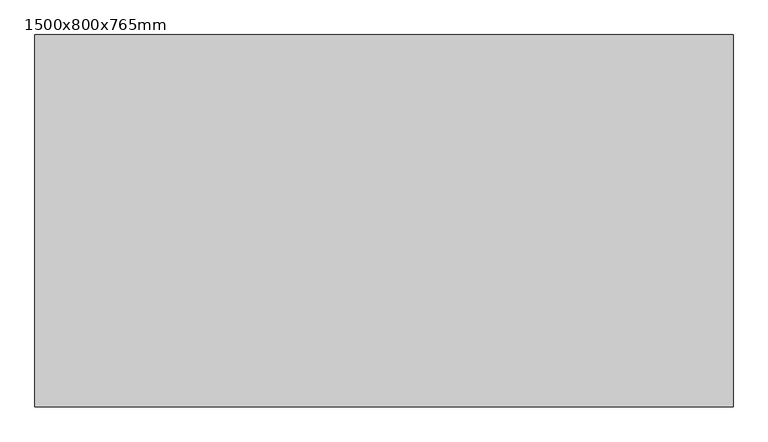
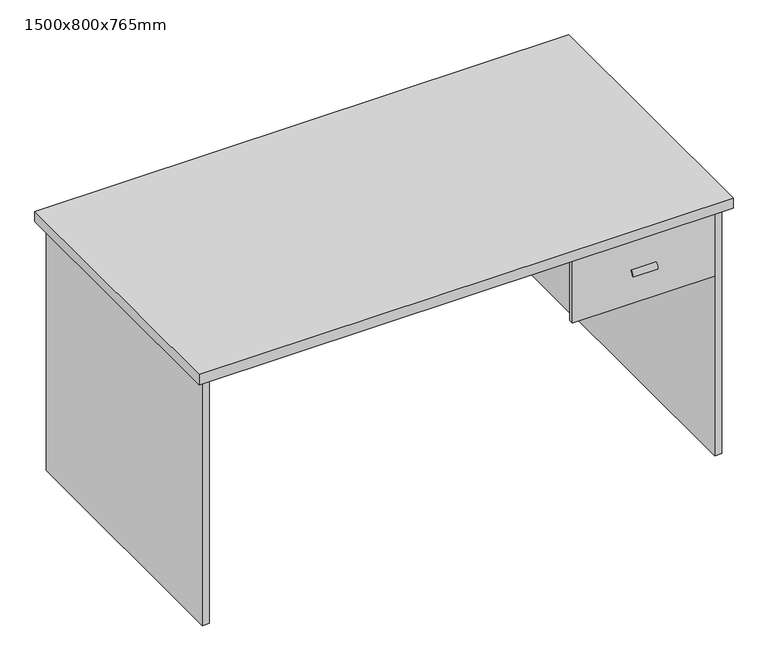
"""IFC4 building model written with IfcOpenShell, lengths in millimetres: furniture geometry, NBS_OffcDsks_OfficeDeskWithDrawer : 1500x800x765mm."""

from ifc_helpers import new_model, si_unit, point, frame, frame_2d, origin, origin_with_axes, place, context, project, spatial, polyline, circle_curve, trimmed, segment, composite_curve, outline, extrude, source, transform, mapped, element, save


def furniture_1500x800x765mm_9c7e9ddd(model_context):
    return source(origin(), model_context, "Body", "SweptSolid", [
        extrude(outline(polyline([(710.0, -380.0), (310.0, -380.0), (310.0, -368.0), (710.0, -368.0), (710.0, -380.0)])), frame((0.0, 0.0, 535.0), z_axis=(0.0, 0.0, 1.0), x_axis=(1.0, 0.0, 0.0)), (0.0, 0.0, 1.0), 200.0),
        extrude(outline(polyline([(698.0, 60.0), (698.0, -368.0), (321.9992987, -368.0), (321.9992987, 60.0), (698.0, 60.0)])), frame((0.0, 0.0, 540.7416159), z_axis=(0.0, 0.0, 1.0), x_axis=(1.0, 0.0, 0.0)), (0.0, 0.0, 1.0), 194.2583841),
        extrude(outline(polyline([(710.0, 380.0), (710.0, 360.0), (-710.0, 360.0), (-710.0, 380.0), (710.0, 380.0)])), frame((0.0, 0.0, 185.0), z_axis=(0.0, 0.0, 1.0), x_axis=(1.0, 0.0, 0.0)), (0.0, 0.0, 1.0), 550.0),
        extrude(outline(polyline([(-710.0, 380.0), (-710.0, -380.0), (-730.0, -380.0), (-730.0, 380.0), (-710.0, 380.0)])), origin_with_axes(), (0.0, 0.0, 1.0), 735.0),
        extrude(outline(polyline([(730.0, 380.0), (730.0, -380.0), (710.0, -380.0), (710.0, 380.0), (730.0, 380.0)])), origin_with_axes(), (0.0, 0.0, 1.0), 735.0),
        extrude(outline(polyline([(750.0, 400.0), (750.0, -400.0), (-750.0, -400.0), (-750.0, 400.0), (750.0, 400.0)])), frame((0.0, 0.0, 735.0), z_axis=(0.0, 0.0, 1.0), x_axis=(1.0, 0.0, 0.0)), (0.0, 0.0, 1.0), 30.0),
        extrude(outline(composite_curve([segment(trimmed(circle_curve(frame_2d((-369.1756558, 618.6602663)), 20.2222385), [point((-389.3776536, 619.5648197))], [point((-380.0, 635.7416159))], False, "CARTESIAN"), True, "CONTINUOUS"), segment(polyline([(-380.0, 635.7416159), (-380.0, 631.5709177)]), True, "CONTINUOUS"), segment(trimmed(circle_curve(frame_2d((-367.0301873, 617.1513707)), 19.394313), [point((-380.0, 631.5709177))], [point((-384.452251, 625.6725838))], True, "CARTESIAN"), True, "CONTINUOUS"), segment(trimmed(circle_curve(frame_2d((-393.0621605, 627.5759127)), 8.8177776), [point((-384.452251, 625.6725838))], [point((-389.3776536, 619.5648197))], False, "CARTESIAN"), True, "CONTINUOUS")], self_intersect=False)), frame((475.0, 0.0, 0.0), z_axis=(1.0, 0.0, 0.0), x_axis=(0.0, 1.0, 0.0)), (0.0, 0.0, 1.0), 70.0),
    ])


if __name__ == "__main__":
    model = new_model("IFC4")
    model_context = context("Model", 3, world=origin())
    ifc_project = project(units=[si_unit("LENGTHUNIT", "METRE", prefix="MILLI")], contexts=[model_context])
    site = spatial("IfcSite", under=ifc_project)
    building = spatial("IfcBuilding", under=site)
    placement = place(None, origin())
    furniture_1500x800x765mm_shape = furniture_1500x800x765mm_9c7e9ddd(model_context)
    element("IfcFurniture", 1, ObjectType="NBS_OffcDsks_OfficeDeskWithDrawer : 1500x800x765mm", at=placement, inside=building, context=model_context, shape_type="MappedRepresentation", body=[
        mapped(furniture_1500x800x765mm_shape, transform((0.0, 0.0, 0.0), x_axis=(1.0, 0.0, 0.0), y_axis=(0.0, 1.0, 0.0), z_axis=(0.0, 0.0, 1.0))),
    ])
    save(model, "model.ifc")

# Revit data of these elements
# Type "NBS_OffcDsks_OfficeDeskWithDrawer : 1500x800x765mm"
#   Type IfcGUID = "2u0XNFrAPALBFZCv81fq27"
#   WarrantyStartDate [instance default] = "1900-12-31T23:59:59"
#   WarrantyGuarantorParts = "n/a"
#   WarrantyGuarantorLabor = "n/a"
#   WarrantyDurationUnit = "year"
#   WarrantyDurationParts = "n/a"
#   WarrantyDurationLabor = "n/a"
#   WarrantyDescription = "n/a"
#   Version = "2"
#   Uniclass2015Version = "Products v1.9"
#   Uniclass2015Title = "Office desks"
#   Uniclass2015Code = "Pr_40_50_21_59"
#   URL = "www.nationalbimlibrary.com"
#   TagNumber [instance default] = "n/a"
#   SustainabilityPerformance = "n/a"
#   Style = "n/a"
#   Size = "1500 x 800 x 765 mm"
#   Shape = "n/a"
#   SerialNumber [instance default] = "n/a"
#   Revision = "n/a"
#   ReplacementCost = "n/a"
#   ProductInformation = "www.nationalbimlibrary.com"
#   OmniClassVersion = "Table 22 2012-05-16"
#   OmniClassTitle = "Office Tables"
#   OmniClassCode = "22-12 51 23"
#   Name = "OfficeDesks_OfficeDeskWithDrawer"
#   NBSReference = "45-35-20/335"
#   NBSDescription = "Office desks"
#   NBSCertification = "www.nationalbimlibrary.com/cert/b4qdjtam"
#   ModelReference = "Office Desk with Drawer"
#   ModelNumber = "n/a"
#   Model = "Office Desk with Drawer"
#   Material = "n/a"
#   ManufacturerURL = "n/a"
#   ManufacturerName = "n/a"
#   Manufacturer = "info@theNBS.com"
#   MainColor = "n/a"
#   InstallationDate [instance default] = "1900-12-31T23:59:59"
#   IfcExportType = "DESK"
#   IfcExportAs = "IfcFurnitureType"
#   Grade = "n/a"
#   Finish = "n/a"
#   Features = "n/a"
#   ExpectedLife = "n/a"
#   DurationUnit = "year"
#   Description = "Generic rectangular office desk with drawer"
#   Constituents = "n/a"
#   Color = "n/a"
#   CodePerformance = "n/a"
#   Category = "Pr_40_50_21_59:Office desks"
#   BarCode [instance default] = "n/a"
#   BIMObjectName = "NBS_OfficeDesks_OfficeDeskWithDrawer"
#   Author = "NBS"
#   AssetType = "Movable"
#   AssetIdentifier [instance default] = "n/a"
#   AccessibilityPerformance = "n/a"
#   WorksurfaceArea = 104.051405 m²
#   NominalWidth = 0.8 m
#   NominalHeight = 0.765 m
#   DesktopThickness = 0.03 m
#   NominalLength = 1.5 m
#   NominalDepth = 0.8 m
#   DrawerFaceWidth = 0.4 m
#   DrawerFaceHeight = 0.2 m
#   DeskLegThickness = 0.02 m
#   DeskLegOffset = 0.02 m
#   DrawerLength = 0.44 m
#   DeskBackDrop = 0.55 m
#   HandleMaterial = NBS_Concept
#   DrawerMaterial = NBS_Concept
#   DesktopMaterial = NBS_Concept
#   DeskSupportMaterial = NBS_Concept
#   Default Elevation = 0
#   Cost = 0
# Element 1 (IfcFurniture, "NBS_OffcDsks_OfficeDeskWithDrawer : 1500x800x765mm")
#   Materials on its faces: "NBS_Concept"
# Materials
#   "NBS_Concept": class "Generic", colour RGB 255 255 255, transparency 0, Description = "To be specified", Cost = 0
